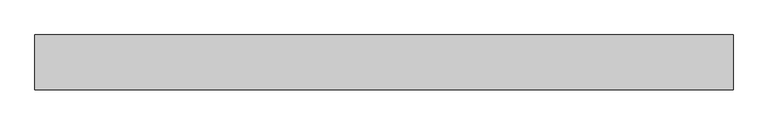
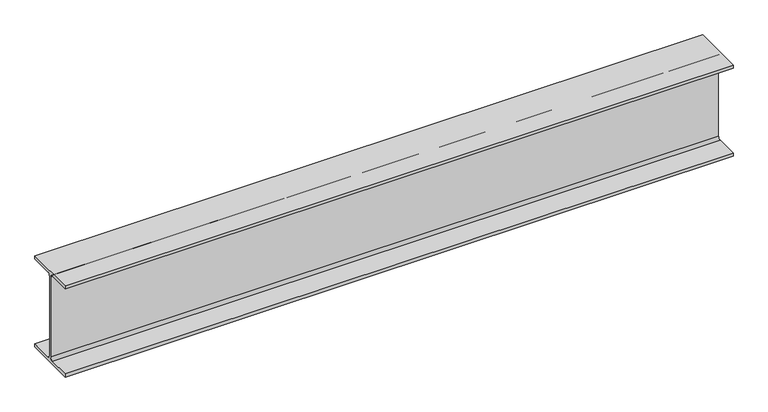
"""IFC4 building model written with IfcOpenShell, lengths in millimetres: beam geometry, Old_Steel Beam_H-KSD3502 : H_SB_ASB_H-194×150x6x9."""

from ifc_helpers import new_model, si_unit, point, frame, frame_2d, origin, place, context, project, spatial, polyline, circle_curve, trimmed, segment, composite_curve, outline, extrude, source, transform, mapped, element, save


def beam_ddb07c81(model_context):
    return source(origin(), model_context, "Body", "SweptSolid", [
        extrude(outline(composite_curve([segment(polyline([(82.5, -141.5), (82.5, -151.7), (-82.5, -151.7), (-82.5, -141.5), (-11.9, -141.5)]), True, "CONTINUOUS"), segment(trimmed(circle_curve(frame_2d((-11.9, -132.6)), 8.9), [point((-11.9, -141.5))], [point((-3.0, -132.6))], True, "CARTESIAN"), True, "CONTINUOUS"), segment(polyline([(-3.0, -132.6), (-3.0, 132.6)]), True, "CONTINUOUS"), segment(trimmed(circle_curve(frame_2d((-11.9, 132.6)), 8.9), [point((-3.0, 132.6))], [point((-11.9, 141.5))], True, "CARTESIAN"), True, "CONTINUOUS"), segment(polyline([(-11.9, 141.5), (-82.5, 141.5), (-82.5, 151.7), (82.5, 151.7), (82.5, 141.5), (11.9, 141.5)]), True, "CONTINUOUS"), segment(trimmed(circle_curve(frame_2d((11.9, 132.6)), 8.9), [point((11.9, 141.5))], [point((3.0, 132.6))], True, "CARTESIAN"), True, "CONTINUOUS"), segment(polyline([(3.0, 132.6), (3.0, -132.6)]), True, "CONTINUOUS"), segment(trimmed(circle_curve(frame_2d((11.9, -132.6)), 8.9), [point((3.0, -132.6))], [point((11.9, -141.5))], True, "CARTESIAN"), True, "CONTINUOUS"), segment(polyline([(11.9, -141.5), (82.5, -141.5)]), True, "CONTINUOUS")], self_intersect=False)), frame((-1203.5869577, 0.0, 0.0), z_axis=(1.0, 0.0, 0.0), x_axis=(0.0, 1.0, 0.0)), (0.0, 0.0, 1.0), 2098.5037314),
    ])


if __name__ == "__main__":
    model = new_model("IFC4")
    model_context = context("Model", 3, world=origin())
    ifc_project = project(units=[si_unit("LENGTHUNIT", "METRE", prefix="MILLI")], contexts=[model_context])
    site = spatial("IfcSite", under=ifc_project)
    building = spatial("IfcBuilding", under=site)
    placement = place(None, origin())
    beam_shape = beam_ddb07c81(model_context)
    element("IfcBeam", 1, ObjectType="Old_Steel Beam_H-KSD3502 : H_SB_ASB_H-194×150x6x9", at=placement, inside=building, context=model_context, shape_type="MappedRepresentation", body=[
        mapped(beam_shape, transform((0.0, 0.0, 0.0), x_axis=(1.0, 0.0, 0.0), y_axis=(0.0, 1.0, 0.0), z_axis=(0.0, 0.0, 1.0))),
    ])
    save(model, "model.ifc")

# Revit data of these elements
# Type "Old_Steel Beam_H-KSD3502 : H_SB_ASB_H-194×150x6x9"
#   Width = 15.0 cm
#   Web Thickness = 0.6 cm
#   Web Fillet = 1.3 cm
#   Warping Constant = 43316.0 cm⁶
#   Torsional Moment of Inertia = 8.622 cm⁴
#   Torsional Modulus = 1.0 cm³
#   Section Area = 39.01 cm²
#   Plastic Modulus weak axis = 104.0 cm³
#   Plastic Modulus strong axis = 309.0 cm³
#   Perimeter = 0.95 m²/m
#   Nominal Weight = 30.60 kgf/m
#   Moment of Inertia weak axis = 507.00 cm⁴
#   Moment of Inertia strong axis = 2690.00 cm⁴
#   Height = 19.4 cm
#   Flange Thickness = 0.9 cm
#   Elastic Modulus weak axis = 67.6 cm³
#   Elastic Modulus strong axis = 277.0 cm³
#   Centroid Vertical = 9.7 cm
#   Centroid Horizontal = 7.5 cm
#   Length [instance default] = 1.5240 m
#   Structural Material [instance default] = Steel, 45-345
#   Assembly Code = ""
# Element 1 (IfcBeam, "Old_Steel Beam_H-KSD3502 : H_SB_ASB_H-194×150x6x9")
#   Structural Material = none
# Materials
#   "Steel, 45-345": class "Metal", colour RGB 189 187 185, transparency 0, Description = "Steel 345 MPa", Cost = 0
